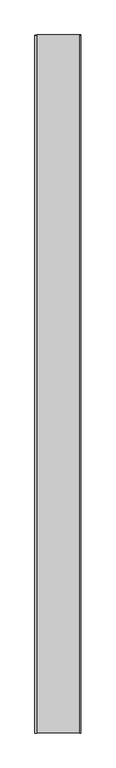
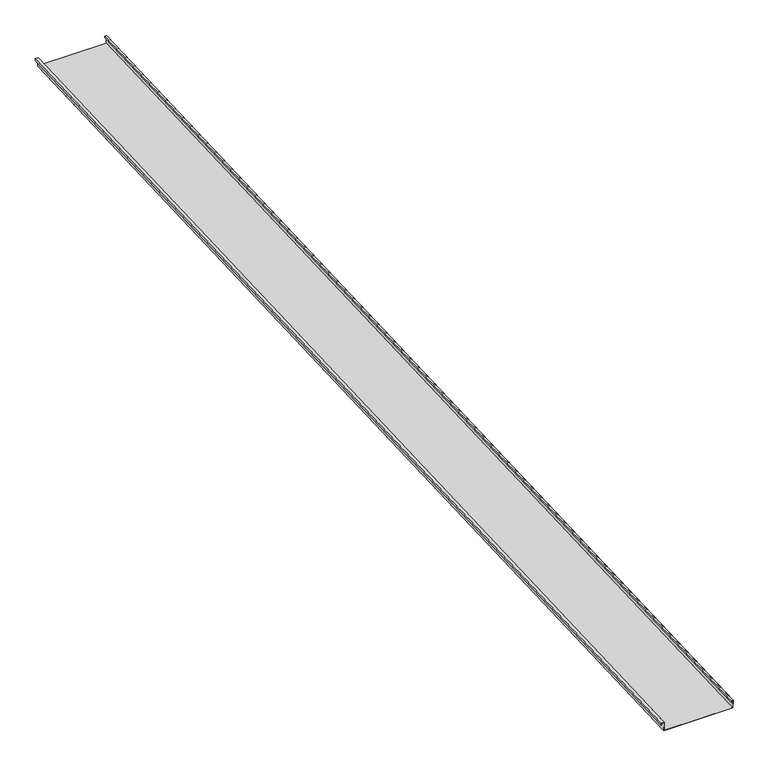
"""IFC4 building model written with IfcOpenShell, lengths in millimetres: proxy geometry, Generic Models 2:Generic Models 2:310765:Generic Models 2:310765 : Generic Models 2:Generic Models 2:310765:104 : Generic Models 2:Generic Models 2:310765:Generic Models 2:310765 : Generic Models 2:Generic Models 2:310765:300385."""

from ifc_helpers import new_model, si_unit, frame, origin, place, context, project, spatial, polyline, outline, extrude, source, transform, mapped, element, save


def generic_models_4d558ed3(model_context):
    return source(origin(), model_context, "Body", "SweptSolid", [
        extrude(outline(polyline([(1.5875, 0.0), (1.5875, 50.8), (407.9875, 50.8), (407.9875, 1.5875), (396.875, 1.5875), (396.875, 11.1125), (398.4625, 11.1125), (398.4625, 3.175), (406.4, 3.175), (406.4, 49.2125), (3.175, 49.2125), (3.175, -1.5874999), (-14.2875, -1.5874999), (-14.2875, 9.525), (-12.7, 9.525), (-12.7, 0.0), (1.5875, 0.0)])), frame((611510.9429739, -581354.4345603, 3902.6697972), z_axis=(0.0, 0.9991330730923568, 0.041630544712067834), x_axis=(1.0, 0.0, 0.0)), (0.0, 0.0, 1.0), 6400.8),
    ])


if __name__ == "__main__":
    model = new_model("IFC4")
    model_context = context("Model", 3, world=origin())
    ifc_project = project(units=[si_unit("LENGTHUNIT", "METRE", prefix="MILLI")], contexts=[model_context])
    site = spatial("IfcSite", under=ifc_project)
    building = spatial("IfcBuilding", under=site)
    placement = place(None, origin())
    generic_models_shape = generic_models_4d558ed3(model_context)
    element("IfcBuildingElementProxy", 1, Name="Generic Models 2:Generic Models 2:310765:Generic Models 2:310765 : Generic Models 2:Generic Models 2:310765:104 : Generic Models 2:Generic Models 2:310765:Generic Models 2:310765 : Generic Models 2:Generic Models 2:310765:300385", ObjectType="Generic Models 2:Generic Models 2:310765:Generic Models 2:310765 : Generic Models 2:Generic Models 2:310765:104 : Generic Models 2:Generic Models 2:310765:Generic Models 2:310765 : Generic Models 2:Generic Models 2:310765:300385", at=placement, inside=building, context=model_context, shape_type="MappedRepresentation", body=[
        mapped(generic_models_shape, transform((0.0, 0.0, 0.0), x_axis=(1.0, 0.0, 0.0), y_axis=(0.0, 1.0, 0.0), z_axis=(0.0, 0.0, 1.0))),
    ])
    save(model, "model.ifc")

# Revit data of these elements
# Type "Generic Models 2:Generic Models 2:310765:Generic Models 2:310765 : Generic Models 2:Generic Models 2:310765:104 : Generic Models 2:Generic Models 2:310765:Generic Models 2:310765 : Generic Models 2:Generic Models 2:310765:300385"
#   NameOverride = "Generic Models 2:Generic Models 2:310765:Generic Models 2:310765 : Generic Models 2:Generic Models 2:310765:300385"
#   ObjectTypeOverride = "Generic Models 2:310765 : Generic Models 2:Generic Models 2:310765"
#   Reference = "Generic Models 2"
#   Tag = "300385"
# Element 1 (IfcBuildingElementProxy, "Generic Models 2:Generic Models 2:310765:Generic Models 2:310765 : Generic Models 2:Generic Models 2:310765:104 : Generic Models 2:Generic Models 2:310765:Generic Models 2:310765 : Generic Models 2:Generic Models 2:310765:300385")
#   Materials on its faces: "THERMAL BROKEN ALUMINUM STOREFRONT FOR POLYCARBONATE"
# Materials
#   "THERMAL BROKEN ALUMINUM STOREFRONT FOR POLYCARBONATE": class "Unassigned", colour RGB 244 244 244, transparency 0, Keynote = "M07611300.01", Cost = 0
